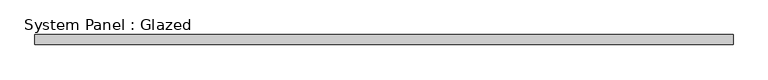
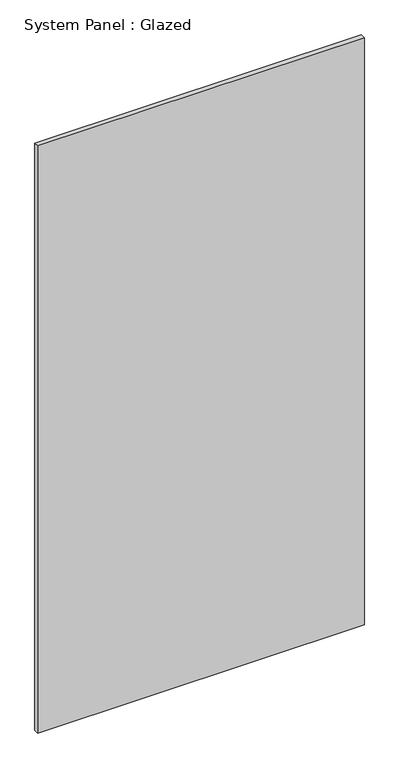
"""IFC4 building model written with IfcOpenShell, lengths in millimetres: plate geometry, System Panel : Glazed."""

from ifc_helpers import new_model, si_unit, origin, origin_with_axes, place, context, project, spatial, polyline, outline, extrude, source, transform, mapped, element, save


def system_panel_glazed_00caa3d2(model_context):
    return source(origin(), model_context, "Body", "SweptSolid", [
        extrude(outline(polyline([(882.65, 19.05), (-882.65, 19.05), (-882.65, 44.45), (882.65, 44.45), (882.65, 19.05)])), origin_with_axes(), (0.0, 0.0, 1.0), 3352.8),
    ])


if __name__ == "__main__":
    model = new_model("IFC4")
    model_context = context("Model", 3, world=origin())
    ifc_project = project(units=[si_unit("LENGTHUNIT", "METRE", prefix="MILLI")], contexts=[model_context])
    site = spatial("IfcSite", under=ifc_project)
    building = spatial("IfcBuilding", under=site)
    placement = place(None, origin())
    system_panel_glazed_shape = system_panel_glazed_00caa3d2(model_context)
    element("IfcPlate", 1, ObjectType="System Panel : Glazed", at=placement, inside=building, context=model_context, shape_type="MappedRepresentation", body=[
        mapped(system_panel_glazed_shape, transform((0.0, 0.0, 0.0), x_axis=(1.0, 0.0, 0.0), y_axis=(0.0, 1.0, 0.0), z_axis=(0.0, 0.0, 1.0))),
    ])
    save(model, "model.ifc")

# Revit data of these elements
# Type "System Panel : Glazed"
#   Construction Type Id = "GSP4R"
#   Analytic Construction = "1/8 in Pilkington single glazing"
#   Visual Light Transmittance = 0.9
#   Solar Heat Gain Coefficient = 0.86
#   Heat Transfer Coefficient (U) = 1.18115 BTU/(h·ft²·°F)
#   Define Thermal Properties by = 1
# Element 1 (IfcPlate, "System Panel : Glazed")
#   Materials on its faces: "Glass"
# Materials
#   "Glass": class "Glass", colour RGB 0 128 192, transparency 0.75, Description = "Soda Lime Glass", Cost = 0
